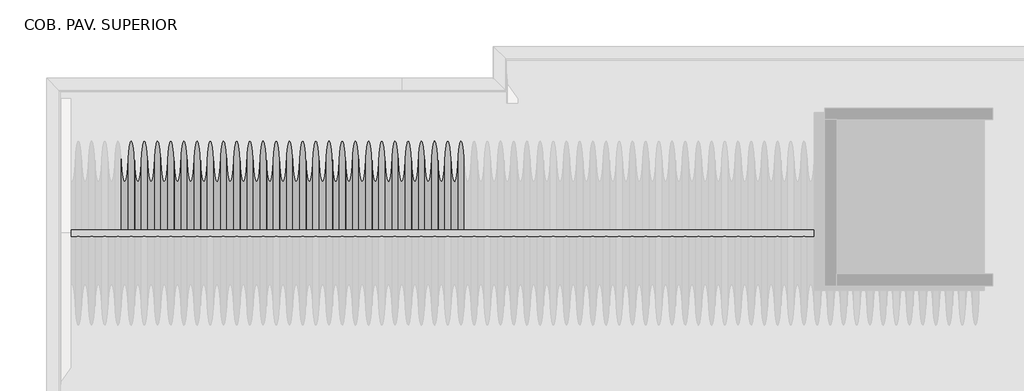
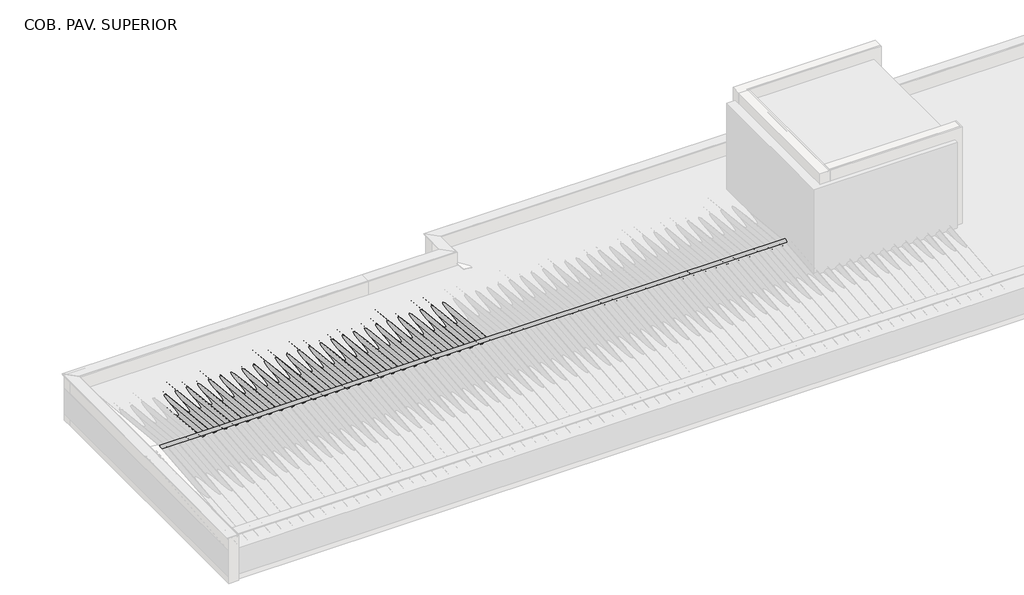
# One storey, part 4 of 8: 36 beams, 8 columns.
"""IFC4 building model written with IfcOpenShell, lengths in millimetres."""

import ifcopenshell
import ifcopenshell.guid

model = None  # the IFC model being written
_history = None  # IfcOwnerHistory: only IFC2X3 demands one
_inside = {}  # id of a spatial element -> (the spatial element, [elements in it])
_under = {}  # id of a project, library or spatial element -> (it, [spatial elements below it])
_declared = {}  # id of a project -> (the project, [libraries it declares])
_typed = {}  # id of a type object -> (the type object, [elements of that type])
_made_of = {}  # id of a material, layer set ... -> (it, [elements and type objects made of it])


def new_model(schema):
    """Start an empty IFC model of exactly this schema.

    Asked for "IFC4X3", IfcOpenShell would pick the latest addendum, in which some entities
    have other attributes; the version numbers below select the first issue.
    IFC2X3 requires an IfcOwnerHistory on every rooted entity: one is made here for all.
    """
    global model, _history
    if schema == "IFC4X3":
        model = ifcopenshell.file(schema_version=(4, 3, 0, 0))
    else:
        model = ifcopenshell.file(schema=schema)
    _inside.clear()
    _under.clear()
    _declared.clear()
    _typed.clear()
    _made_of.clear()
    _history = None
    if model.schema == "IFC2X3":
        org = make("IfcOrganization", Name="unknown")
        user = make(
            "IfcPersonAndOrganization",
            ThePerson=make("IfcPerson", FamilyName="unknown"),
            TheOrganization=org,
        )
        app = make(
            "IfcApplication",
            ApplicationDeveloper=org,
            Version="unknown",
            ApplicationFullName="unknown",
            ApplicationIdentifier="unknown",
        )
        _history = make(
            "IfcOwnerHistory",
            OwningUser=user,
            OwningApplication=app,
            ChangeAction="ADDED",
            CreationDate=0,
        )
    return model


def make(cls, **values):
    """One entity of the class cls with the attributes given. An attribute that is None is left unset."""
    return model.create_entity(
        cls, **{name: value for name, value in values.items() if value is not None}
    )


def rooted(cls, **values):
    """An entity with a GlobalId (a new one), such as an element, a storey or a relation."""
    return make(cls, GlobalId=ifcopenshell.guid.new(), OwnerHistory=_history, **values)


def si_unit(unit_type, name, prefix=None):
    """IfcSIUnit, for example si_unit("LENGTHUNIT", "METRE", prefix="MILLI")."""
    return make("IfcSIUnit", UnitType=unit_type, Prefix=prefix, Name=name)


def assignment(units):
    """IfcUnitAssignment: the units of a project."""
    return None if units is None else make("IfcUnitAssignment", Units=units)


def point(xyz):
    """IfcCartesianPoint."""
    return None if xyz is None else make("IfcCartesianPoint", Coordinates=xyz)


def direction(xyz):
    """IfcDirection."""
    return None if xyz is None else make("IfcDirection", DirectionRatios=xyz)


def frame(location, z_axis=None, x_axis=None):
    """IfcAxis2Placement3D, a coordinate frame: its origin and axes. An axis left out is left unset."""
    return make(
        "IfcAxis2Placement3D",
        Location=point(location),
        Axis=direction(z_axis),
        RefDirection=direction(x_axis),
    )


def frame_2d(location, x_axis=None):
    """IfcAxis2Placement2D, a coordinate frame in the plane: its origin and x axis."""
    return make(
        "IfcAxis2Placement2D", Location=point(location), RefDirection=direction(x_axis)
    )


def origin():
    """The frame at (0, 0, 0) with its axes left unset."""
    return frame((0.0, 0.0, 0.0))


def place(relative_to, where):
    """IfcLocalPlacement: puts the frame where relative to a parent placement (None: the world)."""
    return make(
        "IfcLocalPlacement", PlacementRelTo=relative_to, RelativePlacement=where
    )


def context(
    kind, dimensions, precision=None, world=None, true_north=None, identifier=None
):
    """IfcGeometricRepresentationContext, for example the 3D "Model" context."""
    return make(
        "IfcGeometricRepresentationContext",
        ContextIdentifier=identifier,
        ContextType=kind,
        CoordinateSpaceDimension=dimensions,
        Precision=precision,
        WorldCoordinateSystem=world,
        TrueNorth=true_north,
    )


def project(units=None, contexts=None):
    """IfcProject with its units and contexts."""
    return rooted(
        "IfcProject",
        Name="project",
        RepresentationContexts=contexts,
        UnitsInContext=assignment(units),
    )


def spatial(cls, under=None, at=None, **own):
    """A site, building, storey or space (cls), placed at a placement, below another one or the project."""
    s = rooted(cls, ObjectPlacement=at, **own)
    if under is not None:
        _under.setdefault(under.id(), (under, []))[1].append(s)
    return s


def polyline(points):
    """IfcPolyline through the points."""
    return make("IfcPolyline", Points=[point(p) for p in points])


def circle_curve(where, radius):
    """IfcCircle in the frame where."""
    return make("IfcCircle", Position=where, Radius=radius)


def trimmed(basis, trim1, trim2, sense, master):
    """IfcTrimmedCurve: the piece of a basis curve between two trims."""
    return make(
        "IfcTrimmedCurve",
        BasisCurve=basis,
        Trim1=trim1,
        Trim2=trim2,
        SenseAgreement=sense,
        MasterRepresentation=master,
    )


def segment(curve, same_sense, transition):
    """IfcCompositeCurveSegment."""
    return make(
        "IfcCompositeCurveSegment",
        Transition=transition,
        SameSense=same_sense,
        ParentCurve=curve,
    )


def composite_curve(segments, self_intersect=None):
    """IfcCompositeCurve: segments joined end to end."""
    return make("IfcCompositeCurve", Segments=segments, SelfIntersect=self_intersect)


def outline(outer, holes=None, kind="AREA"):
    """IfcArbitraryClosedProfileDef: a profile drawn as a closed curve; with holes, ...WithVoids."""
    if holes is None:
        return make("IfcArbitraryClosedProfileDef", ProfileType=kind, OuterCurve=outer)
    return make(
        "IfcArbitraryProfileDefWithVoids",
        ProfileType=kind,
        OuterCurve=outer,
        InnerCurves=holes,
    )


def extrude(swept, where, along, depth):
    """IfcExtrudedAreaSolid: the profile swept, set in the frame where, extruded along a direction by depth."""
    return make(
        "IfcExtrudedAreaSolid",
        SweptArea=swept,
        Position=where,
        ExtrudedDirection=direction(along),
        Depth=depth,
    )


def shape(context_of_items, identifier, shape_type, items):
    """IfcShapeRepresentation: the items that make up one representation, for example the "Body"."""
    return make(
        "IfcShapeRepresentation",
        ContextOfItems=context_of_items,
        RepresentationIdentifier=identifier,
        RepresentationType=shape_type,
        Items=items,
    )


def source(mapping_origin, context_of_items, identifier, shape_type, items):
    """IfcRepresentationMap: a shape defined once, which mapped items show again and again."""
    return make(
        "IfcRepresentationMap",
        MappingOrigin=mapping_origin,
        MappedRepresentation=shape(context_of_items, identifier, shape_type, items),
    )


def transform(
    local_origin,
    x_axis=None,
    y_axis=None,
    z_axis=None,
    scale=None,
    scale2=None,
    scale3=None,
    uniform=True,
):
    """IfcCartesianTransformationOperator3D, or its non-uniform kind. x_axis, y_axis, z_axis: its Axis1, 2, 3."""
    if uniform:
        return make(
            "IfcCartesianTransformationOperator3D",
            Axis1=direction(x_axis),
            Axis2=direction(y_axis),
            LocalOrigin=point(local_origin),
            Scale=scale,
            Axis3=direction(z_axis),
        )
    return make(
        "IfcCartesianTransformationOperator3DnonUniform",
        Axis1=direction(x_axis),
        Axis2=direction(y_axis),
        LocalOrigin=point(local_origin),
        Scale=scale,
        Axis3=direction(z_axis),
        Scale2=scale2,
        Scale3=scale3,
    )


def mapped(mapping_source, mapping_target):
    """IfcMappedItem: shows the shape of a source again, moved by a transform."""
    return make(
        "IfcMappedItem", MappingSource=mapping_source, MappingTarget=mapping_target
    )


def made_of(thing, what):
    """Note that an element or type object is made of a material, layer set ...; save() writes the relation."""
    if what is not None:
        _made_of.setdefault(what.id(), (what, []))[1].append(thing)
    return thing


def element(
    cls,
    number,
    at=None,
    inside=None,
    cuts=None,
    type_object=None,
    material=None,
    context=None,
    identifier="Body",
    shape_type=None,
    held_by="IfcProductDefinitionShape",
    body=None,
    shapes=None,
    **own,
):
    """One element of the class cls, such as IfcWall. Its Tag is "e" and its number.

    at: its placement. inside: the storey or other place that contains it. cuts: it is an
    opening in that element (IfcRelVoidsElement). A single representation is given by context,
    identifier, shape_type and body (its items); several are given by shapes. held_by: the class
    of the entity that holds the representations. save() writes the other relations.
    """
    e = rooted(cls, Tag="e%d" % number, ObjectPlacement=at, **own)
    if body is not None:
        shapes = [shape(context, identifier, shape_type, body)]
    if shapes is not None:
        e.Representation = make(held_by, Representations=shapes)
    if inside is not None:
        _inside.setdefault(inside.id(), (inside, []))[1].append(e)
    if cuts is not None:
        rooted(
            "IfcRelVoidsElement", RelatingBuildingElement=cuts, RelatedOpeningElement=e
        )
    if type_object is not None:
        _typed.setdefault(type_object.id(), (type_object, []))[1].append(e)
    return made_of(e, material)


def aggregate(whole, parts):
    """IfcRelAggregates: a whole, such as a stair, and the parts it consists of."""
    return rooted("IfcRelAggregates", RelatingObject=whole, RelatedObjects=parts)


def save(model, path):
    """Write the relations noted so far, then the file.

    IfcRelAggregates (storeys below a building ...), IfcRelContainedInSpatialStructure (elements
    in a storey), IfcRelDefinesByType, IfcRelAssociatesMaterial and IfcRelDeclares: one each for
    every whole, place, type object, material and project.
    """
    for whole, parts in _under.values():
        aggregate(whole, parts)
    for where, things in _inside.values():
        rooted(
            "IfcRelContainedInSpatialStructure",
            RelatedElements=things,
            RelatingStructure=where,
        )
    for kind, things in _typed.values():
        rooted("IfcRelDefinesByType", RelatedObjects=things, RelatingType=kind)
    for what, things in _made_of.values():
        rooted("IfcRelAssociatesMaterial", RelatedObjects=things, RelatingMaterial=what)
    for by, libraries in _declared.values():
        rooted("IfcRelDeclares", RelatingContext=by, RelatedDefinitions=libraries)
    model.write(path)


def beam_fe4ddbad(model_context):
    return source(origin(), model_context, "Body", "SweptSolid", [
        extrude(outline(polyline([(998.8971968, 30.0), (998.8971968, -30.0), (-998.8971974, -30.0), (-998.8971974, 30.0), (998.8971968, 30.0)])), frame((0.0, 0.0, -60.0), z_axis=(0.0, 0.0, 1.0), x_axis=(1.0, 0.0, 0.0)), (0.0, 0.0, 1.0), 120.0),
    ])


def cumeeira_telha_ondulada_fibrocimento_80a8fd81(model_context):
    return source(origin(), model_context, "Body", "SweptSolid", [
        extrude(outline(composite_curve([segment(polyline([(58.3970135, 42.4437972), (53.9055884, 40.2467307)]), True, "CONTINUOUS"), segment(trimmed(circle_curve(frame_2d((-1.6029865, 13.0936483)), 61.7939461), [point((53.9055884, 40.2467307))], [point((-57.1115615, 40.2467307))], True, "CARTESIAN"), True, "CONTINUOUS"), segment(polyline([(-57.1115615, 40.2467307), (-61.6029865, 42.4437972)]), True, "CONTINUOUS"), segment(trimmed(circle_curve(frame_2d((-1.6029865, 13.0936483)), 66.7939461), [point((-61.6029865, 42.4437972))], [point((58.3970135, 42.4437972))], False, "CARTESIAN"), True, "CONTINUOUS")], self_intersect=False)), frame((-7085.3584094, 0.0, 0.0), z_axis=(1.0, 0.0, 0.0), x_axis=(0.0, 1.0, 0.0)), (0.0, 0.0, 1.0), 14170.7168187),
    ])


def viga_cumeeira_6x16cm_bb341ce4(model_context):
    return source(origin(), model_context, "Body", "SweptSolid", [
        extrude(outline(polyline([(7083.3, 30.0), (7083.3, -30.0), (-7082.5, -30.0), (-7082.5, 30.0), (7083.3, 30.0)])), frame((0.0, 0.0, -80.0), z_axis=(0.0, 0.0, 1.0), x_axis=(1.0, 0.0, 0.0)), (0.0, 0.0, 1.0), 160.0),
    ])


def column_6c15bf79(model_context):
    return source(origin(), model_context, "Body", "SweptSolid", [
        extrude(outline(polyline([(30.0, 80.0), (30.0, -80.0), (-30.0, -80.0), (-30.0, 80.0), (30.0, 80.0)])), frame((0.0, 0.0, 6710.0), z_axis=(0.0, 0.0, 1.0), x_axis=(1.0, 0.0, 0.0)), (0.0, 0.0, 1.0), 467.5),
    ])


def column_1adb463a(model_context):
    return source(origin(), model_context, "Body", "SweptSolid", [
        extrude(outline(polyline([(30.0, 80.0), (30.0, -80.0), (-30.0, -80.0), (-30.0, 80.0), (30.0, 80.0)])), frame((0.0, 0.0, 6710.0), z_axis=(0.0, 0.0, 1.0), x_axis=(1.0, 0.0, 0.0)), (0.0, 0.0, 1.0), 284.6),
    ])


def column_910cb117(model_context):
    return source(origin(), model_context, "Body", "SweptSolid", [
        extrude(outline(polyline([(30.0, 80.0), (30.0, -80.0), (-30.0, -80.0), (-30.0, 80.0), (30.0, 80.0)])), frame((0.0, 0.0, 6710.0), z_axis=(0.0, 0.0, 1.0), x_axis=(1.0, 0.0, 0.0)), (0.0, 0.0, 1.0), 371.3),
    ])


model = new_model("IFC4")

# Units and contexts
model_context = context("Model", 3, world=origin())
ifc_project = project(units=[si_unit("LENGTHUNIT", "METRE", prefix="MILLI")], contexts=[model_context])

# Site, building, storey
site = spatial("IfcSite", under=ifc_project)
building = spatial("IfcBuilding", under=site)
storey = spatial("IfcBuildingStorey", under=building, Name="COB. PAV. SUPERIOR", Elevation=6650.0)

# Beams
placement = place(None, origin())
beam_shape = beam_fe4ddbad(model_context)
element("IfcBeam", 1, ObjectType="Madeira de lei : Berço 6x12cm", at=placement, inside=storey, context=model_context, shape_type="MappedRepresentation", body=[
    mapped(beam_shape, transform((-11738.1841096, -6365.3711004, 6680.0), x_axis=(1.0, 0.0, 0.0), y_axis=(0.0, 0.0, -1.0), z_axis=(0.0, 1.0, 0.0))),
])
element("IfcBeam", 2, ObjectType="Madeira de lei : Berço 6x12cm", at=placement, inside=storey, context=model_context, shape_type="MappedRepresentation", body=[
    mapped(beam_shape, transform((-11738.1841096, -5498.3211004, 6680.0), x_axis=(1.0, 0.0, 0.0), y_axis=(0.0, 0.0, -1.0), z_axis=(0.0, 1.0, 0.0))),
])
element("IfcBeam", 3, ObjectType="Madeira de lei : Berço 6x12cm", at=placement, inside=storey, context=model_context, shape_type="MappedRepresentation", body=[
    mapped(beam_shape, transform((-9740.3897147, -7777.6209418, 6680.0), x_axis=(1.0, 0.0, 0.0), y_axis=(0.0, 0.0, -1.0), z_axis=(0.0, 1.0, 0.0))),
])
element("IfcBeam", 4, ObjectType="Madeira de lei : Berço 6x12cm", at=placement, inside=storey, context=model_context, shape_type="MappedRepresentation", body=[
    mapped(beam_shape, transform((-7742.5953199, -7777.6209418, 6680.0), x_axis=(1.0, 0.0, 0.0), y_axis=(0.0, 0.0, -1.0), z_axis=(0.0, 1.0, 0.0))),
])
element("IfcBeam", 5, ObjectType="Madeira de lei : Berço 6x12cm", at=placement, inside=storey, context=model_context, shape_type="MappedRepresentation", body=[
    mapped(beam_shape, transform((-5744.8009251, -7777.6209418, 6680.0), x_axis=(1.0, 0.0, 0.0), y_axis=(0.0, 0.0, -1.0), z_axis=(0.0, 1.0, 0.0))),
])
element("IfcBeam", 6, ObjectType="Madeira de lei : Berço 6x12cm", at=placement, inside=storey, context=model_context, shape_type="MappedRepresentation", body=[
    mapped(beam_shape, transform((-9740.3897147, -6365.3711004, 6680.0), x_axis=(1.0, 0.0, 0.0), y_axis=(0.0, 0.0, -1.0), z_axis=(0.0, 1.0, 0.0))),
])
element("IfcBeam", 7, ObjectType="Madeira de lei : Berço 6x12cm", at=placement, inside=storey, context=model_context, shape_type="MappedRepresentation", body=[
    mapped(beam_shape, transform((-7742.5953199, -6365.3711004, 6680.0), x_axis=(1.0, 0.0, 0.0), y_axis=(0.0, 0.0, -1.0), z_axis=(0.0, 1.0, 0.0))),
])
element("IfcBeam", 8, ObjectType="Madeira de lei : Berço 6x12cm", at=placement, inside=storey, context=model_context, shape_type="MappedRepresentation", body=[
    mapped(beam_shape, transform((-9740.3897147, -5498.3211004, 6680.0), x_axis=(1.0, 0.0, 0.0), y_axis=(0.0, 0.0, -1.0), z_axis=(0.0, 1.0, 0.0))),
])
cumeeira_telha_ondulada_fibrocimento_shape = cumeeira_telha_ondulada_fibrocimento_80a8fd81(model_context)
element("IfcBeam", 9, ObjectType="Cumeeira Telha Ondulada : Fibrocimento", at=placement, inside=storey, context=model_context, shape_type="MappedRepresentation", body=[
    mapped(cumeeira_telha_ondulada_fibrocimento_shape, transform((-5656.9228976, -7777.6209418, 7375.6251229), x_axis=(-1.0, 0.0, 0.0), y_axis=(0.0, -1.0, 0.0), z_axis=(0.0, 0.0, 1.0))),
])
element("IfcBeam", 10, ObjectType="Telha Ondulada : Fibrocimento", at=placement, inside=storey, context=model_context, shape_type="SweptSolid", body=[
    extrude(outline(composite_curve([segment(trimmed(circle_curve(frame_2d((-58.7002978, -53.2060539)), 66.7939461), [point((-29.3501489, 6.7939461))], [point((-29.3501489, -113.2060539))], False, "CARTESIAN"), True, "CONTINUOUS"), segment(polyline([(-29.3501489, -113.2060539), (-31.5472154, -108.7146289)]), True, "CONTINUOUS"), segment(trimmed(circle_curve(frame_2d((-58.7002978, -53.2060539)), 61.7939461), [point((-31.5472154, -108.7146289))], [point((-31.5472154, 2.3025211))], True, "CARTESIAN"), True, "CONTINUOUS"), segment(trimmed(circle_curve(frame_2d((0.0, 66.7939461)), 71.7939461), [point((-31.5472154, 2.3025211))], [point((-31.5472154, 131.2853711))], False, "CARTESIAN"), True, "CONTINUOUS"), segment(polyline([(-31.5472154, 131.2853711), (-29.3501489, 126.7939461)]), True, "CONTINUOUS"), segment(trimmed(circle_curve(frame_2d((0.0, 66.7939461)), 66.7939461), [point((-29.3501489, 126.7939461))], [point((-29.3501489, 6.7939461))], True, "CARTESIAN"), True, "CONTINUOUS")], self_intersect=False)), frame((-11474.7843743, -5298.1805671, 7164.3215886), z_axis=(0.0, -0.9950371902099894, 0.0995037190209978), x_axis=(0.0, 0.0995037190209978, 0.9950371902099894)), (0.0, 0.0, 1.0), 2482.5761317),
])
element("IfcBeam", 11, ObjectType="Telha Ondulada : Fibrocimento", at=placement, inside=storey, context=model_context, shape_type="SweptSolid", body=[
    extrude(outline(composite_curve([segment(trimmed(circle_curve(frame_2d((-58.7002978, -53.2060539)), 66.7939461), [point((-29.3501489, 6.7939461))], [point((-29.3501489, -113.2060539))], False, "CARTESIAN"), True, "CONTINUOUS"), segment(polyline([(-29.3501489, -113.2060539), (-31.5472154, -108.7146289)]), True, "CONTINUOUS"), segment(trimmed(circle_curve(frame_2d((-58.7002978, -53.2060539)), 61.7939461), [point((-31.5472154, -108.7146289))], [point((-31.5472154, 2.3025211))], True, "CARTESIAN"), True, "CONTINUOUS"), segment(trimmed(circle_curve(frame_2d((0.0, 66.7939461)), 71.7939461), [point((-31.5472154, 2.3025211))], [point((-31.5472154, 131.2853711))], False, "CARTESIAN"), True, "CONTINUOUS"), segment(polyline([(-31.5472154, 131.2853711), (-29.3501489, 126.7939461)]), True, "CONTINUOUS"), segment(trimmed(circle_curve(frame_2d((0.0, 66.7939461)), 66.7939461), [point((-29.3501489, 126.7939461))], [point((-29.3501489, 6.7939461))], True, "CARTESIAN"), True, "CONTINUOUS")], self_intersect=False)), frame((-11230.2843743, -5298.1805671, 7164.3215886), z_axis=(0.0, -0.9950371902099894, 0.0995037190209978), x_axis=(0.0, 0.0995037190209978, 0.9950371902099894)), (0.0, 0.0, 1.0), 2482.5761317),
])
element("IfcBeam", 12, ObjectType="Telha Ondulada : Fibrocimento", at=placement, inside=storey, context=model_context, shape_type="SweptSolid", body=[
    extrude(outline(composite_curve([segment(trimmed(circle_curve(frame_2d((-58.7002978, -53.2060539)), 66.7939461), [point((-29.3501489, 6.7939461))], [point((-29.3501489, -113.2060539))], False, "CARTESIAN"), True, "CONTINUOUS"), segment(polyline([(-29.3501489, -113.2060539), (-31.5472154, -108.7146289)]), True, "CONTINUOUS"), segment(trimmed(circle_curve(frame_2d((-58.7002978, -53.2060539)), 61.7939461), [point((-31.5472154, -108.7146289))], [point((-31.5472154, 2.3025211))], True, "CARTESIAN"), True, "CONTINUOUS"), segment(trimmed(circle_curve(frame_2d((0.0, 66.7939461)), 71.7939461), [point((-31.5472154, 2.3025211))], [point((-31.5472154, 131.2853711))], False, "CARTESIAN"), True, "CONTINUOUS"), segment(polyline([(-31.5472154, 131.2853711), (-29.3501489, 126.7939461)]), True, "CONTINUOUS"), segment(trimmed(circle_curve(frame_2d((0.0, 66.7939461)), 66.7939461), [point((-29.3501489, 126.7939461))], [point((-29.3501489, 6.7939461))], True, "CARTESIAN"), True, "CONTINUOUS")], self_intersect=False)), frame((-10985.7843743, -5298.1805671, 7164.3215886), z_axis=(0.0, -0.9950371902099894, 0.09950371902099785), x_axis=(0.0, 0.09950371902099785, 0.9950371902099894)), (0.0, 0.0, 1.0), 2482.5761317),
])
element("IfcBeam", 13, ObjectType="Telha Ondulada : Fibrocimento", at=placement, inside=storey, context=model_context, shape_type="SweptSolid", body=[
    extrude(outline(composite_curve([segment(trimmed(circle_curve(frame_2d((-58.7002978, -53.2060539)), 66.7939461), [point((-29.3501489, 6.7939461))], [point((-29.3501489, -113.2060539))], False, "CARTESIAN"), True, "CONTINUOUS"), segment(polyline([(-29.3501489, -113.2060539), (-31.5472154, -108.7146289)]), True, "CONTINUOUS"), segment(trimmed(circle_curve(frame_2d((-58.7002978, -53.2060539)), 61.7939461), [point((-31.5472154, -108.7146289))], [point((-31.5472154, 2.3025211))], True, "CARTESIAN"), True, "CONTINUOUS"), segment(trimmed(circle_curve(frame_2d((0.0, 66.7939461)), 71.7939461), [point((-31.5472154, 2.3025211))], [point((-31.5472154, 131.2853711))], False, "CARTESIAN"), True, "CONTINUOUS"), segment(polyline([(-31.5472154, 131.2853711), (-29.3501489, 126.7939461)]), True, "CONTINUOUS"), segment(trimmed(circle_curve(frame_2d((0.0, 66.7939461)), 66.7939461), [point((-29.3501489, 126.7939461))], [point((-29.3501489, 6.7939461))], True, "CARTESIAN"), True, "CONTINUOUS")], self_intersect=False)), frame((-10741.2843743, -5298.1805671, 7164.3215886), z_axis=(0.0, -0.9950371902099894, 0.09950371902099785), x_axis=(0.0, 0.09950371902099785, 0.9950371902099894)), (0.0, 0.0, 1.0), 2482.5761317),
])
element("IfcBeam", 14, ObjectType="Telha Ondulada : Fibrocimento", at=placement, inside=storey, context=model_context, shape_type="SweptSolid", body=[
    extrude(outline(composite_curve([segment(trimmed(circle_curve(frame_2d((-58.7002978, -53.2060539)), 66.7939461), [point((-29.3501489, 6.7939461))], [point((-29.3501489, -113.2060539))], False, "CARTESIAN"), True, "CONTINUOUS"), segment(polyline([(-29.3501489, -113.2060539), (-31.5472154, -108.7146289)]), True, "CONTINUOUS"), segment(trimmed(circle_curve(frame_2d((-58.7002978, -53.2060539)), 61.7939461), [point((-31.5472154, -108.7146289))], [point((-31.5472154, 2.3025211))], True, "CARTESIAN"), True, "CONTINUOUS"), segment(trimmed(circle_curve(frame_2d((0.0, 66.7939461)), 71.7939461), [point((-31.5472154, 2.3025211))], [point((-31.5472154, 131.2853711))], False, "CARTESIAN"), True, "CONTINUOUS"), segment(polyline([(-31.5472154, 131.2853711), (-29.3501489, 126.7939461)]), True, "CONTINUOUS"), segment(trimmed(circle_curve(frame_2d((0.0, 66.7939461)), 66.7939461), [point((-29.3501489, 126.7939461))], [point((-29.3501489, 6.7939461))], True, "CARTESIAN"), True, "CONTINUOUS")], self_intersect=False)), frame((-10496.7843743, -5298.1805671, 7164.3215886), z_axis=(0.0, -0.9950371902099894, 0.09950371902099785), x_axis=(0.0, 0.09950371902099785, 0.9950371902099894)), (0.0, 0.0, 1.0), 2482.5761317),
])
element("IfcBeam", 15, ObjectType="Telha Ondulada : Fibrocimento", at=placement, inside=storey, context=model_context, shape_type="SweptSolid", body=[
    extrude(outline(composite_curve([segment(trimmed(circle_curve(frame_2d((-58.7002978, -53.2060539)), 66.7939461), [point((-29.3501489, 6.7939461))], [point((-29.3501489, -113.2060539))], False, "CARTESIAN"), True, "CONTINUOUS"), segment(polyline([(-29.3501489, -113.2060539), (-31.5472154, -108.7146289)]), True, "CONTINUOUS"), segment(trimmed(circle_curve(frame_2d((-58.7002978, -53.2060539)), 61.7939461), [point((-31.5472154, -108.7146289))], [point((-31.5472154, 2.3025211))], True, "CARTESIAN"), True, "CONTINUOUS"), segment(trimmed(circle_curve(frame_2d((0.0, 66.7939461)), 71.7939461), [point((-31.5472154, 2.3025211))], [point((-31.5472154, 131.2853711))], False, "CARTESIAN"), True, "CONTINUOUS"), segment(polyline([(-31.5472154, 131.2853711), (-29.3501489, 126.7939461)]), True, "CONTINUOUS"), segment(trimmed(circle_curve(frame_2d((0.0, 66.7939461)), 66.7939461), [point((-29.3501489, 126.7939461))], [point((-29.3501489, 6.7939461))], True, "CARTESIAN"), True, "CONTINUOUS")], self_intersect=False)), frame((-10252.2843743, -5298.1805671, 7164.3215886), z_axis=(0.0, -0.9950371902099894, 0.09950371902099785), x_axis=(0.0, 0.09950371902099785, 0.9950371902099894)), (0.0, 0.0, 1.0), 2482.5761317),
])
element("IfcBeam", 16, ObjectType="Telha Ondulada : Fibrocimento", at=placement, inside=storey, context=model_context, shape_type="SweptSolid", body=[
    extrude(outline(composite_curve([segment(trimmed(circle_curve(frame_2d((-58.7002978, -53.2060539)), 66.7939461), [point((-29.3501489, 6.7939461))], [point((-29.3501489, -113.2060539))], False, "CARTESIAN"), True, "CONTINUOUS"), segment(polyline([(-29.3501489, -113.2060539), (-31.5472154, -108.7146289)]), True, "CONTINUOUS"), segment(trimmed(circle_curve(frame_2d((-58.7002978, -53.2060539)), 61.7939461), [point((-31.5472154, -108.7146289))], [point((-31.5472154, 2.3025211))], True, "CARTESIAN"), True, "CONTINUOUS"), segment(trimmed(circle_curve(frame_2d((0.0, 66.7939461)), 71.7939461), [point((-31.5472154, 2.3025211))], [point((-31.5472154, 131.2853711))], False, "CARTESIAN"), True, "CONTINUOUS"), segment(polyline([(-31.5472154, 131.2853711), (-29.3501489, 126.7939461)]), True, "CONTINUOUS"), segment(trimmed(circle_curve(frame_2d((0.0, 66.7939461)), 66.7939461), [point((-29.3501489, 126.7939461))], [point((-29.3501489, 6.7939461))], True, "CARTESIAN"), True, "CONTINUOUS")], self_intersect=False)), frame((-10007.7843743, -5298.1805671, 7164.3215886), z_axis=(0.0, -0.9950371902099894, 0.09950371902099785), x_axis=(0.0, 0.09950371902099785, 0.9950371902099894)), (0.0, 0.0, 1.0), 2482.5761317),
])
element("IfcBeam", 17, ObjectType="Telha Ondulada : Fibrocimento", at=placement, inside=storey, context=model_context, shape_type="SweptSolid", body=[
    extrude(outline(composite_curve([segment(trimmed(circle_curve(frame_2d((-58.7002978, -53.2060539)), 66.7939461), [point((-29.3501489, 6.7939461))], [point((-29.3501489, -113.2060539))], False, "CARTESIAN"), True, "CONTINUOUS"), segment(polyline([(-29.3501489, -113.2060539), (-31.5472154, -108.7146289)]), True, "CONTINUOUS"), segment(trimmed(circle_curve(frame_2d((-58.7002978, -53.2060539)), 61.7939461), [point((-31.5472154, -108.7146289))], [point((-31.5472154, 2.3025211))], True, "CARTESIAN"), True, "CONTINUOUS"), segment(trimmed(circle_curve(frame_2d((0.0, 66.7939461)), 71.7939461), [point((-31.5472154, 2.3025211))], [point((-31.5472154, 131.2853711))], False, "CARTESIAN"), True, "CONTINUOUS"), segment(polyline([(-31.5472154, 131.2853711), (-29.3501489, 126.7939461)]), True, "CONTINUOUS"), segment(trimmed(circle_curve(frame_2d((0.0, 66.7939461)), 66.7939461), [point((-29.3501489, 126.7939461))], [point((-29.3501489, 6.7939461))], True, "CARTESIAN"), True, "CONTINUOUS")], self_intersect=False)), frame((-9763.2843743, -5298.1805671, 7164.3215886), z_axis=(0.0, -0.9950371902099894, 0.09950371902099785), x_axis=(0.0, 0.09950371902099785, 0.9950371902099894)), (0.0, 0.0, 1.0), 2482.5761317),
])
element("IfcBeam", 18, ObjectType="Telha Ondulada : Fibrocimento", at=placement, inside=storey, context=model_context, shape_type="SweptSolid", body=[
    extrude(outline(composite_curve([segment(trimmed(circle_curve(frame_2d((-58.7002978, -53.2060539)), 66.7939461), [point((-29.3501489, 6.7939461))], [point((-29.3501489, -113.2060539))], False, "CARTESIAN"), True, "CONTINUOUS"), segment(polyline([(-29.3501489, -113.2060539), (-31.5472154, -108.7146289)]), True, "CONTINUOUS"), segment(trimmed(circle_curve(frame_2d((-58.7002978, -53.2060539)), 61.7939461), [point((-31.5472154, -108.7146289))], [point((-31.5472154, 2.3025211))], True, "CARTESIAN"), True, "CONTINUOUS"), segment(trimmed(circle_curve(frame_2d((0.0, 66.7939461)), 71.7939461), [point((-31.5472154, 2.3025211))], [point((-31.5472154, 131.2853711))], False, "CARTESIAN"), True, "CONTINUOUS"), segment(polyline([(-31.5472154, 131.2853711), (-29.3501489, 126.7939461)]), True, "CONTINUOUS"), segment(trimmed(circle_curve(frame_2d((0.0, 66.7939461)), 66.7939461), [point((-29.3501489, 126.7939461))], [point((-29.3501489, 6.7939461))], True, "CARTESIAN"), True, "CONTINUOUS")], self_intersect=False)), frame((-9518.7843743, -5298.1805671, 7164.3215886), z_axis=(0.0, -0.9950371902099894, 0.09950371902099785), x_axis=(0.0, 0.09950371902099785, 0.9950371902099894)), (0.0, 0.0, 1.0), 2482.5761317),
])
element("IfcBeam", 19, ObjectType="Telha Ondulada : Fibrocimento", at=placement, inside=storey, context=model_context, shape_type="SweptSolid", body=[
    extrude(outline(composite_curve([segment(trimmed(circle_curve(frame_2d((-58.7002978, -53.2060539)), 66.7939461), [point((-29.3501489, 6.7939461))], [point((-29.3501489, -113.2060539))], False, "CARTESIAN"), True, "CONTINUOUS"), segment(polyline([(-29.3501489, -113.2060539), (-31.5472154, -108.7146289)]), True, "CONTINUOUS"), segment(trimmed(circle_curve(frame_2d((-58.7002978, -53.2060539)), 61.7939461), [point((-31.5472154, -108.7146289))], [point((-31.5472154, 2.3025211))], True, "CARTESIAN"), True, "CONTINUOUS"), segment(trimmed(circle_curve(frame_2d((0.0, 66.7939461)), 71.7939461), [point((-31.5472154, 2.3025211))], [point((-31.5472154, 131.2853711))], False, "CARTESIAN"), True, "CONTINUOUS"), segment(polyline([(-31.5472154, 131.2853711), (-29.3501489, 126.7939461)]), True, "CONTINUOUS"), segment(trimmed(circle_curve(frame_2d((0.0, 66.7939461)), 66.7939461), [point((-29.3501489, 126.7939461))], [point((-29.3501489, 6.7939461))], True, "CARTESIAN"), True, "CONTINUOUS")], self_intersect=False)), frame((-9274.2843743, -5298.1805671, 7164.3215886), z_axis=(0.0, -0.9950371902099894, 0.09950371902099785), x_axis=(0.0, 0.09950371902099785, 0.9950371902099894)), (0.0, 0.0, 1.0), 2482.5761317),
])
element("IfcBeam", 20, ObjectType="Telha Ondulada : Fibrocimento", at=placement, inside=storey, context=model_context, shape_type="SweptSolid", body=[
    extrude(outline(composite_curve([segment(trimmed(circle_curve(frame_2d((-58.7002978, -53.2060539)), 66.7939461), [point((-29.3501489, 6.7939461))], [point((-29.3501489, -113.2060539))], False, "CARTESIAN"), True, "CONTINUOUS"), segment(polyline([(-29.3501489, -113.2060539), (-31.5472154, -108.7146289)]), True, "CONTINUOUS"), segment(trimmed(circle_curve(frame_2d((-58.7002978, -53.2060539)), 61.7939461), [point((-31.5472154, -108.7146289))], [point((-31.5472154, 2.3025211))], True, "CARTESIAN"), True, "CONTINUOUS"), segment(trimmed(circle_curve(frame_2d((0.0, 66.7939461)), 71.7939461), [point((-31.5472154, 2.3025211))], [point((-31.5472154, 131.2853711))], False, "CARTESIAN"), True, "CONTINUOUS"), segment(polyline([(-31.5472154, 131.2853711), (-29.3501489, 126.7939461)]), True, "CONTINUOUS"), segment(trimmed(circle_curve(frame_2d((0.0, 66.7939461)), 66.7939461), [point((-29.3501489, 126.7939461))], [point((-29.3501489, 6.7939461))], True, "CARTESIAN"), True, "CONTINUOUS")], self_intersect=False)), frame((-9029.7843743, -5298.1805671, 7164.3215886), z_axis=(0.0, -0.9950371902099894, 0.09950371902099785), x_axis=(0.0, 0.09950371902099785, 0.9950371902099894)), (0.0, 0.0, 1.0), 2482.5761317),
])
element("IfcBeam", 21, ObjectType="Telha Ondulada : Fibrocimento", at=placement, inside=storey, context=model_context, shape_type="SweptSolid", body=[
    extrude(outline(composite_curve([segment(trimmed(circle_curve(frame_2d((-58.7002978, -53.2060539)), 66.7939461), [point((-29.3501489, 6.7939461))], [point((-29.3501489, -113.2060539))], False, "CARTESIAN"), True, "CONTINUOUS"), segment(polyline([(-29.3501489, -113.2060539), (-31.5472154, -108.7146289)]), True, "CONTINUOUS"), segment(trimmed(circle_curve(frame_2d((-58.7002978, -53.2060539)), 61.7939461), [point((-31.5472154, -108.7146289))], [point((-31.5472154, 2.3025211))], True, "CARTESIAN"), True, "CONTINUOUS"), segment(trimmed(circle_curve(frame_2d((0.0, 66.7939461)), 71.7939461), [point((-31.5472154, 2.3025211))], [point((-31.5472154, 131.2853711))], False, "CARTESIAN"), True, "CONTINUOUS"), segment(polyline([(-31.5472154, 131.2853711), (-29.3501489, 126.7939461)]), True, "CONTINUOUS"), segment(trimmed(circle_curve(frame_2d((0.0, 66.7939461)), 66.7939461), [point((-29.3501489, 126.7939461))], [point((-29.3501489, 6.7939461))], True, "CARTESIAN"), True, "CONTINUOUS")], self_intersect=False)), frame((-8785.2843743, -5298.1805671, 7164.3215886), z_axis=(0.0, -0.9950371902099894, 0.09950371902099785), x_axis=(0.0, 0.09950371902099785, 0.9950371902099894)), (0.0, 0.0, 1.0), 2482.5761317),
])
element("IfcBeam", 22, ObjectType="Telha Ondulada : Fibrocimento", at=placement, inside=storey, context=model_context, shape_type="SweptSolid", body=[
    extrude(outline(composite_curve([segment(trimmed(circle_curve(frame_2d((-58.7002978, -53.2060539)), 66.7939461), [point((-29.3501489, 6.7939461))], [point((-29.3501489, -113.2060539))], False, "CARTESIAN"), True, "CONTINUOUS"), segment(polyline([(-29.3501489, -113.2060539), (-31.5472154, -108.7146289)]), True, "CONTINUOUS"), segment(trimmed(circle_curve(frame_2d((-58.7002978, -53.2060539)), 61.7939461), [point((-31.5472154, -108.7146289))], [point((-31.5472154, 2.3025211))], True, "CARTESIAN"), True, "CONTINUOUS"), segment(trimmed(circle_curve(frame_2d((0.0, 66.7939461)), 71.7939461), [point((-31.5472154, 2.3025211))], [point((-31.5472154, 131.2853711))], False, "CARTESIAN"), True, "CONTINUOUS"), segment(polyline([(-31.5472154, 131.2853711), (-29.3501489, 126.7939461)]), True, "CONTINUOUS"), segment(trimmed(circle_curve(frame_2d((0.0, 66.7939461)), 66.7939461), [point((-29.3501489, 126.7939461))], [point((-29.3501489, 6.7939461))], True, "CARTESIAN"), True, "CONTINUOUS")], self_intersect=False)), frame((-8540.7843743, -5298.1805671, 7164.3215886), z_axis=(0.0, -0.9950371902099894, 0.09950371902099785), x_axis=(0.0, 0.09950371902099785, 0.9950371902099894)), (0.0, 0.0, 1.0), 2482.5761317),
])
element("IfcBeam", 23, ObjectType="Telha Ondulada : Fibrocimento", at=placement, inside=storey, context=model_context, shape_type="SweptSolid", body=[
    extrude(outline(composite_curve([segment(trimmed(circle_curve(frame_2d((-58.7002978, -53.2060539)), 66.7939461), [point((-29.3501489, 6.7939461))], [point((-29.3501489, -113.2060539))], False, "CARTESIAN"), True, "CONTINUOUS"), segment(polyline([(-29.3501489, -113.2060539), (-31.5472154, -108.7146289)]), True, "CONTINUOUS"), segment(trimmed(circle_curve(frame_2d((-58.7002978, -53.2060539)), 61.7939461), [point((-31.5472154, -108.7146289))], [point((-31.5472154, 2.3025211))], True, "CARTESIAN"), True, "CONTINUOUS"), segment(trimmed(circle_curve(frame_2d((0.0, 66.7939461)), 71.7939461), [point((-31.5472154, 2.3025211))], [point((-31.5472154, 131.2853711))], False, "CARTESIAN"), True, "CONTINUOUS"), segment(polyline([(-31.5472154, 131.2853711), (-29.3501489, 126.7939461)]), True, "CONTINUOUS"), segment(trimmed(circle_curve(frame_2d((0.0, 66.7939461)), 66.7939461), [point((-29.3501489, 126.7939461))], [point((-29.3501489, 6.7939461))], True, "CARTESIAN"), True, "CONTINUOUS")], self_intersect=False)), frame((-8296.2843743, -5298.1805671, 7164.3215886), z_axis=(0.0, -0.9950371902099894, 0.09950371902099785), x_axis=(0.0, 0.09950371902099785, 0.9950371902099894)), (0.0, 0.0, 1.0), 2482.5761317),
])
element("IfcBeam", 24, ObjectType="Telha Ondulada : Fibrocimento", at=placement, inside=storey, context=model_context, shape_type="SweptSolid", body=[
    extrude(outline(composite_curve([segment(trimmed(circle_curve(frame_2d((-58.7002978, -53.2060539)), 66.7939461), [point((-29.3501489, 6.7939461))], [point((-29.3501489, -113.2060539))], False, "CARTESIAN"), True, "CONTINUOUS"), segment(polyline([(-29.3501489, -113.2060539), (-31.5472154, -108.7146289)]), True, "CONTINUOUS"), segment(trimmed(circle_curve(frame_2d((-58.7002978, -53.2060539)), 61.7939461), [point((-31.5472154, -108.7146289))], [point((-31.5472154, 2.3025211))], True, "CARTESIAN"), True, "CONTINUOUS"), segment(trimmed(circle_curve(frame_2d((0.0, 66.7939461)), 71.7939461), [point((-31.5472154, 2.3025211))], [point((-31.5472154, 131.2853711))], False, "CARTESIAN"), True, "CONTINUOUS"), segment(polyline([(-31.5472154, 131.2853711), (-29.3501489, 126.7939461)]), True, "CONTINUOUS"), segment(trimmed(circle_curve(frame_2d((0.0, 66.7939461)), 66.7939461), [point((-29.3501489, 126.7939461))], [point((-29.3501489, 6.7939461))], True, "CARTESIAN"), True, "CONTINUOUS")], self_intersect=False)), frame((-8051.7843743, -5298.1805671, 7164.3215886), z_axis=(0.0, -0.9950371902099894, 0.0995037190209978), x_axis=(0.0, 0.0995037190209978, 0.9950371902099894)), (0.0, 0.0, 1.0), 2482.5761317),
])
element("IfcBeam", 25, ObjectType="Telha Ondulada : Fibrocimento", at=placement, inside=storey, context=model_context, shape_type="SweptSolid", body=[
    extrude(outline(composite_curve([segment(trimmed(circle_curve(frame_2d((-58.7002978, -53.2060539)), 66.7939461), [point((-29.3501489, 6.7939461))], [point((-29.3501489, -113.2060539))], False, "CARTESIAN"), True, "CONTINUOUS"), segment(polyline([(-29.3501489, -113.2060539), (-31.5472154, -108.7146289)]), True, "CONTINUOUS"), segment(trimmed(circle_curve(frame_2d((-58.7002978, -53.2060539)), 61.7939461), [point((-31.5472154, -108.7146289))], [point((-31.5472154, 2.3025211))], True, "CARTESIAN"), True, "CONTINUOUS"), segment(trimmed(circle_curve(frame_2d((0.0, 66.7939461)), 71.7939461), [point((-31.5472154, 2.3025211))], [point((-31.5472154, 131.2853711))], False, "CARTESIAN"), True, "CONTINUOUS"), segment(polyline([(-31.5472154, 131.2853711), (-29.3501489, 126.7939461)]), True, "CONTINUOUS"), segment(trimmed(circle_curve(frame_2d((0.0, 66.7939461)), 66.7939461), [point((-29.3501489, 126.7939461))], [point((-29.3501489, 6.7939461))], True, "CARTESIAN"), True, "CONTINUOUS")], self_intersect=False)), frame((-7807.2843743, -5298.1805671, 7164.3215886), z_axis=(0.0, -0.9950371902099894, 0.09950371902099785), x_axis=(0.0, 0.09950371902099785, 0.9950371902099894)), (0.0, 0.0, 1.0), 2482.5761317),
])
element("IfcBeam", 26, ObjectType="Telha Ondulada : Fibrocimento", at=placement, inside=storey, context=model_context, shape_type="SweptSolid", body=[
    extrude(outline(composite_curve([segment(trimmed(circle_curve(frame_2d((-58.7002978, -53.2060539)), 66.7939461), [point((-29.3501489, 6.7939461))], [point((-29.3501489, -113.2060539))], False, "CARTESIAN"), True, "CONTINUOUS"), segment(polyline([(-29.3501489, -113.2060539), (-31.5472154, -108.7146289)]), True, "CONTINUOUS"), segment(trimmed(circle_curve(frame_2d((-58.7002978, -53.2060539)), 61.7939461), [point((-31.5472154, -108.7146289))], [point((-31.5472154, 2.3025211))], True, "CARTESIAN"), True, "CONTINUOUS"), segment(trimmed(circle_curve(frame_2d((0.0, 66.7939461)), 71.7939461), [point((-31.5472154, 2.3025211))], [point((-31.5472154, 131.2853711))], False, "CARTESIAN"), True, "CONTINUOUS"), segment(polyline([(-31.5472154, 131.2853711), (-29.3501489, 126.7939461)]), True, "CONTINUOUS"), segment(trimmed(circle_curve(frame_2d((0.0, 66.7939461)), 66.7939461), [point((-29.3501489, 126.7939461))], [point((-29.3501489, 6.7939461))], True, "CARTESIAN"), True, "CONTINUOUS")], self_intersect=False)), frame((-7562.7843743, -5298.1805671, 7164.3215886), z_axis=(0.0, -0.9950371902099894, 0.09950371902099785), x_axis=(0.0, 0.09950371902099785, 0.9950371902099894)), (0.0, 0.0, 1.0), 2482.5761317),
])
element("IfcBeam", 27, ObjectType="Telha Ondulada : Fibrocimento", at=placement, inside=storey, context=model_context, shape_type="SweptSolid", body=[
    extrude(outline(composite_curve([segment(trimmed(circle_curve(frame_2d((-58.7002979, -53.2060539)), 66.7939461), [point((-29.350149, 6.7939461))], [point((-29.350149, -113.2060539))], False, "CARTESIAN"), True, "CONTINUOUS"), segment(polyline([(-29.350149, -113.2060539), (-31.5472155, -108.7146289)]), True, "CONTINUOUS"), segment(trimmed(circle_curve(frame_2d((-58.7002979, -53.2060539)), 61.7939461), [point((-31.5472155, -108.7146289))], [point((-31.5472155, 2.3025211))], True, "CARTESIAN"), True, "CONTINUOUS"), segment(trimmed(circle_curve(frame_2d((0.0, 66.7939461)), 71.7939461), [point((-31.5472155, 2.3025211))], [point((-31.5472155, 131.2853711))], False, "CARTESIAN"), True, "CONTINUOUS"), segment(polyline([(-31.5472155, 131.2853711), (-29.350149, 126.7939461)]), True, "CONTINUOUS"), segment(trimmed(circle_curve(frame_2d((0.0, 66.7939461)), 66.7939461), [point((-29.350149, 126.7939461))], [point((-29.350149, 6.7939461))], True, "CARTESIAN"), True, "CONTINUOUS")], self_intersect=False)), frame((-7318.2843743, -5447.4361457, 7179.2471465), z_axis=(0.0, -0.9950371902099893, 0.09950371902099792), x_axis=(0.0, 0.09950371902099792, 0.9950371902099893)), (0.0, 0.0, 1.0), 2332.5761317),
])
element("IfcBeam", 28, ObjectType="Telha Ondulada : Fibrocimento", at=placement, inside=storey, context=model_context, shape_type="SweptSolid", body=[
    extrude(outline(composite_curve([segment(trimmed(circle_curve(frame_2d((-58.7002978, -53.2060539)), 66.7939461), [point((-29.3501489, 6.7939461))], [point((-29.3501489, -113.2060539))], False, "CARTESIAN"), True, "CONTINUOUS"), segment(polyline([(-29.3501489, -113.2060539), (-31.5472154, -108.7146289)]), True, "CONTINUOUS"), segment(trimmed(circle_curve(frame_2d((-58.7002978, -53.2060539)), 61.7939461), [point((-31.5472154, -108.7146289))], [point((-31.5472154, 2.3025211))], True, "CARTESIAN"), True, "CONTINUOUS"), segment(trimmed(circle_curve(frame_2d((0.0, 66.7939461)), 71.7939461), [point((-31.5472154, 2.3025211))], [point((-31.5472154, 131.2853711))], False, "CARTESIAN"), True, "CONTINUOUS"), segment(polyline([(-31.5472154, 131.2853711), (-29.3501489, 126.7939461)]), True, "CONTINUOUS"), segment(trimmed(circle_curve(frame_2d((0.0, 66.7939461)), 66.7939461), [point((-29.3501489, 126.7939461))], [point((-29.3501489, 6.7939461))], True, "CARTESIAN"), True, "CONTINUOUS")], self_intersect=False)), frame((-7073.7843743, -5298.1805671, 7164.3215886), z_axis=(0.0, -0.9950371902099894, 0.09950371902099785), x_axis=(0.0, 0.09950371902099785, 0.9950371902099894)), (0.0, 0.0, 1.0), 2482.5761317),
])
element("IfcBeam", 29, ObjectType="Telha Ondulada : Fibrocimento", at=placement, inside=storey, context=model_context, shape_type="SweptSolid", body=[
    extrude(outline(composite_curve([segment(trimmed(circle_curve(frame_2d((-58.7002978, -53.2060539)), 66.7939461), [point((-29.3501489, 6.7939461))], [point((-29.3501489, -113.2060539))], False, "CARTESIAN"), True, "CONTINUOUS"), segment(polyline([(-29.3501489, -113.2060539), (-31.5472154, -108.7146289)]), True, "CONTINUOUS"), segment(trimmed(circle_curve(frame_2d((-58.7002978, -53.2060539)), 61.7939461), [point((-31.5472154, -108.7146289))], [point((-31.5472154, 2.3025211))], True, "CARTESIAN"), True, "CONTINUOUS"), segment(trimmed(circle_curve(frame_2d((0.0, 66.7939461)), 71.7939461), [point((-31.5472154, 2.3025211))], [point((-31.5472154, 131.2853711))], False, "CARTESIAN"), True, "CONTINUOUS"), segment(polyline([(-31.5472154, 131.2853711), (-29.3501489, 126.7939461)]), True, "CONTINUOUS"), segment(trimmed(circle_curve(frame_2d((0.0, 66.7939461)), 66.7939461), [point((-29.3501489, 126.7939461))], [point((-29.3501489, 6.7939461))], True, "CARTESIAN"), True, "CONTINUOUS")], self_intersect=False)), frame((-6829.2843743, -5298.1805671, 7164.3215886), z_axis=(0.0, -0.9950371902099894, 0.09950371902099785), x_axis=(0.0, 0.09950371902099785, 0.9950371902099894)), (0.0, 0.0, 1.0), 2482.5761317),
])
element("IfcBeam", 30, ObjectType="Telha Ondulada : Fibrocimento", at=placement, inside=storey, context=model_context, shape_type="SweptSolid", body=[
    extrude(outline(composite_curve([segment(trimmed(circle_curve(frame_2d((-58.7002978, -53.2060539)), 66.7939461), [point((-29.3501489, 6.7939461))], [point((-29.3501489, -113.2060539))], False, "CARTESIAN"), True, "CONTINUOUS"), segment(polyline([(-29.3501489, -113.2060539), (-31.5472154, -108.7146289)]), True, "CONTINUOUS"), segment(trimmed(circle_curve(frame_2d((-58.7002978, -53.2060539)), 61.7939461), [point((-31.5472154, -108.7146289))], [point((-31.5472154, 2.3025211))], True, "CARTESIAN"), True, "CONTINUOUS"), segment(trimmed(circle_curve(frame_2d((0.0, 66.7939461)), 71.7939461), [point((-31.5472154, 2.3025211))], [point((-31.5472154, 131.2853711))], False, "CARTESIAN"), True, "CONTINUOUS"), segment(polyline([(-31.5472154, 131.2853711), (-29.3501489, 126.7939461)]), True, "CONTINUOUS"), segment(trimmed(circle_curve(frame_2d((0.0, 66.7939461)), 66.7939461), [point((-29.3501489, 126.7939461))], [point((-29.3501489, 6.7939461))], True, "CARTESIAN"), True, "CONTINUOUS")], self_intersect=False)), frame((-6584.7843743, -5298.1805671, 7164.3215886), z_axis=(0.0, -0.9950371902099894, 0.09950371902099785), x_axis=(0.0, 0.09950371902099785, 0.9950371902099894)), (0.0, 0.0, 1.0), 2482.5761317),
])
element("IfcBeam", 31, ObjectType="Telha Ondulada : Fibrocimento", at=placement, inside=storey, context=model_context, shape_type="SweptSolid", body=[
    extrude(outline(composite_curve([segment(trimmed(circle_curve(frame_2d((-58.7002978, -53.2060539)), 66.7939461), [point((-29.3501489, 6.7939461))], [point((-29.3501489, -113.2060539))], False, "CARTESIAN"), True, "CONTINUOUS"), segment(polyline([(-29.3501489, -113.2060539), (-31.5472154, -108.7146289)]), True, "CONTINUOUS"), segment(trimmed(circle_curve(frame_2d((-58.7002978, -53.2060539)), 61.7939461), [point((-31.5472154, -108.7146289))], [point((-31.5472154, 2.3025211))], True, "CARTESIAN"), True, "CONTINUOUS"), segment(trimmed(circle_curve(frame_2d((0.0, 66.7939461)), 71.7939461), [point((-31.5472154, 2.3025211))], [point((-31.5472154, 131.2853711))], False, "CARTESIAN"), True, "CONTINUOUS"), segment(polyline([(-31.5472154, 131.2853711), (-29.3501489, 126.7939461)]), True, "CONTINUOUS"), segment(trimmed(circle_curve(frame_2d((0.0, 66.7939461)), 66.7939461), [point((-29.3501489, 126.7939461))], [point((-29.3501489, 6.7939461))], True, "CARTESIAN"), True, "CONTINUOUS")], self_intersect=False)), frame((-6340.2843743, -5298.1805671, 7164.3215886), z_axis=(0.0, -0.9950371902099894, 0.09950371902099785), x_axis=(0.0, 0.09950371902099785, 0.9950371902099894)), (0.0, 0.0, 1.0), 2482.5761317),
])
element("IfcBeam", 32, ObjectType="Telha Ondulada : Fibrocimento", at=placement, inside=storey, context=model_context, shape_type="SweptSolid", body=[
    extrude(outline(composite_curve([segment(trimmed(circle_curve(frame_2d((-58.7002978, -53.2060539)), 66.7939461), [point((-29.3501489, 6.7939461))], [point((-29.3501489, -113.2060539))], False, "CARTESIAN"), True, "CONTINUOUS"), segment(polyline([(-29.3501489, -113.2060539), (-31.5472154, -108.7146289)]), True, "CONTINUOUS"), segment(trimmed(circle_curve(frame_2d((-58.7002978, -53.2060539)), 61.7939461), [point((-31.5472154, -108.7146289))], [point((-31.5472154, 2.3025211))], True, "CARTESIAN"), True, "CONTINUOUS"), segment(trimmed(circle_curve(frame_2d((0.0, 66.7939461)), 71.7939461), [point((-31.5472154, 2.3025211))], [point((-31.5472154, 131.2853711))], False, "CARTESIAN"), True, "CONTINUOUS"), segment(polyline([(-31.5472154, 131.2853711), (-29.3501489, 126.7939461)]), True, "CONTINUOUS"), segment(trimmed(circle_curve(frame_2d((0.0, 66.7939461)), 66.7939461), [point((-29.3501489, 126.7939461))], [point((-29.3501489, 6.7939461))], True, "CARTESIAN"), True, "CONTINUOUS")], self_intersect=False)), frame((-6095.7843743, -5298.1805671, 7164.3215886), z_axis=(0.0, -0.9950371902099894, 0.09950371902099785), x_axis=(0.0, 0.09950371902099785, 0.9950371902099894)), (0.0, 0.0, 1.0), 2482.5761317),
])
element("IfcBeam", 33, ObjectType="Telha Ondulada : Fibrocimento", at=placement, inside=storey, context=model_context, shape_type="SweptSolid", body=[
    extrude(outline(composite_curve([segment(trimmed(circle_curve(frame_2d((-58.7002978, -53.2060539)), 66.7939461), [point((-29.3501489, 6.7939461))], [point((-29.3501489, -113.2060539))], False, "CARTESIAN"), True, "CONTINUOUS"), segment(polyline([(-29.3501489, -113.2060539), (-31.5472154, -108.7146289)]), True, "CONTINUOUS"), segment(trimmed(circle_curve(frame_2d((-58.7002978, -53.2060539)), 61.7939461), [point((-31.5472154, -108.7146289))], [point((-31.5472154, 2.3025211))], True, "CARTESIAN"), True, "CONTINUOUS"), segment(trimmed(circle_curve(frame_2d((0.0, 66.7939461)), 71.7939461), [point((-31.5472154, 2.3025211))], [point((-31.5472154, 131.2853711))], False, "CARTESIAN"), True, "CONTINUOUS"), segment(polyline([(-31.5472154, 131.2853711), (-29.3501489, 126.7939461)]), True, "CONTINUOUS"), segment(trimmed(circle_curve(frame_2d((0.0, 66.7939461)), 66.7939461), [point((-29.3501489, 126.7939461))], [point((-29.3501489, 6.7939461))], True, "CARTESIAN"), True, "CONTINUOUS")], self_intersect=False)), frame((-5851.2843743, -5298.1805671, 7164.3215886), z_axis=(0.0, -0.9950371902099894, 0.09950371902099785), x_axis=(0.0, 0.09950371902099785, 0.9950371902099894)), (0.0, 0.0, 1.0), 2482.5761317),
])
element("IfcBeam", 34, ObjectType="Telha Ondulada : Fibrocimento", at=placement, inside=storey, context=model_context, shape_type="SweptSolid", body=[
    extrude(outline(composite_curve([segment(trimmed(circle_curve(frame_2d((-58.7002978, -53.2060539)), 66.7939461), [point((-29.3501489, 6.7939461))], [point((-29.3501489, -113.2060539))], False, "CARTESIAN"), True, "CONTINUOUS"), segment(polyline([(-29.3501489, -113.2060539), (-31.5472154, -108.7146289)]), True, "CONTINUOUS"), segment(trimmed(circle_curve(frame_2d((-58.7002978, -53.2060539)), 61.7939461), [point((-31.5472154, -108.7146289))], [point((-31.5472154, 2.3025211))], True, "CARTESIAN"), True, "CONTINUOUS"), segment(trimmed(circle_curve(frame_2d((0.0, 66.7939461)), 71.7939461), [point((-31.5472154, 2.3025211))], [point((-31.5472154, 131.2853711))], False, "CARTESIAN"), True, "CONTINUOUS"), segment(polyline([(-31.5472154, 131.2853711), (-29.3501489, 126.7939461)]), True, "CONTINUOUS"), segment(trimmed(circle_curve(frame_2d((0.0, 66.7939461)), 66.7939461), [point((-29.3501489, 126.7939461))], [point((-29.3501489, 6.7939461))], True, "CARTESIAN"), True, "CONTINUOUS")], self_intersect=False)), frame((-5606.7843743, -5298.1805671, 7164.3215886), z_axis=(0.0, -0.9950371902099894, 0.09950371902099785), x_axis=(0.0, 0.09950371902099785, 0.9950371902099894)), (0.0, 0.0, 1.0), 2482.5761317),
])
element("IfcBeam", 35, ObjectType="Telha Ondulada : Fibrocimento", at=placement, inside=storey, context=model_context, shape_type="SweptSolid", body=[
    extrude(outline(composite_curve([segment(trimmed(circle_curve(frame_2d((-58.7002978, -53.2060539)), 66.7939461), [point((-29.3501489, 6.7939461))], [point((-29.3501489, -113.2060539))], False, "CARTESIAN"), True, "CONTINUOUS"), segment(polyline([(-29.3501489, -113.2060539), (-31.5472154, -108.7146289)]), True, "CONTINUOUS"), segment(trimmed(circle_curve(frame_2d((-58.7002978, -53.2060539)), 61.7939461), [point((-31.5472154, -108.7146289))], [point((-31.5472154, 2.3025211))], True, "CARTESIAN"), True, "CONTINUOUS"), segment(trimmed(circle_curve(frame_2d((0.0, 66.7939461)), 71.7939461), [point((-31.5472154, 2.3025211))], [point((-31.5472154, 131.2853711))], False, "CARTESIAN"), True, "CONTINUOUS"), segment(polyline([(-31.5472154, 131.2853711), (-29.3501489, 126.7939461)]), True, "CONTINUOUS"), segment(trimmed(circle_curve(frame_2d((0.0, 66.7939461)), 66.7939461), [point((-29.3501489, 126.7939461))], [point((-29.3501489, 6.7939461))], True, "CARTESIAN"), True, "CONTINUOUS")], self_intersect=False)), frame((-5362.2843743, -5298.1805671, 7164.3215886), z_axis=(0.0, -0.9950371902099894, 0.09950371902099785), x_axis=(0.0, 0.09950371902099785, 0.9950371902099894)), (0.0, 0.0, 1.0), 2482.5761317),
])
viga_cumeeira_6x16cm_shape = viga_cumeeira_6x16cm_bb341ce4(model_context)
element("IfcBeam", 36, ObjectType="Madeira de lei : Viga Cumeeira 6x16cm", at=placement, inside=storey, context=model_context, shape_type="MappedRepresentation", body=[
    mapped(viga_cumeeira_6x16cm_shape, transform((-5654.581307, -7777.6209418, 7258.0), x_axis=(1.0, 0.0, 0.0), y_axis=(0.0, 1.0, 0.0), z_axis=(0.0, 0.0, 1.0))),
])

# Columns
column_shape = column_6c15bf79(model_context)
element("IfcColumn", 37, ObjectType="Madeira de lei-Coluna : Pontalete 6X16cm", at=placement, inside=storey, context=model_context, shape_type="MappedRepresentation", body=[
    mapped(column_shape, transform((-9738.1841096, -7777.6209418, 0.0), x_axis=(0.0, -1.0, 0.0), y_axis=(1.0, 0.0, 0.0), z_axis=(0.0, 0.0, 1.0))),
])
element("IfcColumn", 38, ObjectType="Madeira de lei-Coluna : Pontalete 6X16cm", at=placement, inside=storey, context=model_context, shape_type="MappedRepresentation", body=[
    mapped(column_shape, transform((-7738.1841096, -7777.6209418, 0.0), x_axis=(0.0, -1.0, 0.0), y_axis=(1.0, 0.0, 0.0), z_axis=(0.0, 0.0, 1.0))),
])
element("IfcColumn", 39, ObjectType="Madeira de lei-Coluna : Pontalete 6X16cm", at=placement, inside=storey, context=model_context, shape_type="MappedRepresentation", body=[
    mapped(column_shape, transform((-5738.1841096, -7777.6209418, 0.0), x_axis=(0.0, -1.0, 0.0), y_axis=(1.0, 0.0, 0.0), z_axis=(0.0, 0.0, 1.0))),
])
column_2_shape = column_1adb463a(model_context)
element("IfcColumn", 40, ObjectType="Madeira de lei-Coluna : Pontalete 6X16cm", at=placement, inside=storey, context=model_context, shape_type="MappedRepresentation", body=[
    mapped(column_2_shape, transform((-11738.1841096, -5498.3211004, 0.0), x_axis=(0.0, -1.0, 0.0), y_axis=(1.0, 0.0, 0.0), z_axis=(0.0, 0.0, 1.0))),
])
element("IfcColumn", 41, ObjectType="Madeira de lei-Coluna : Pontalete 6X16cm", at=placement, inside=storey, context=model_context, shape_type="MappedRepresentation", body=[
    mapped(column_2_shape, transform((-9738.1841096, -5498.3211004, 0.0), x_axis=(0.0, -1.0, 0.0), y_axis=(1.0, 0.0, 0.0), z_axis=(0.0, 0.0, 1.0))),
])
column_3_shape = column_910cb117(model_context)
element("IfcColumn", 42, ObjectType="Madeira de lei-Coluna : Pontalete 6X16cm", at=placement, inside=storey, context=model_context, shape_type="MappedRepresentation", body=[
    mapped(column_3_shape, transform((-11738.1841096, -6365.3711004, 0.0), x_axis=(0.0, -1.0, 0.0), y_axis=(1.0, 0.0, 0.0), z_axis=(0.0, 0.0, 1.0))),
])
element("IfcColumn", 43, ObjectType="Madeira de lei-Coluna : Pontalete 6X16cm", at=placement, inside=storey, context=model_context, shape_type="MappedRepresentation", body=[
    mapped(column_3_shape, transform((-9738.1841096, -6365.3711004, 0.0), x_axis=(0.0, -1.0, 0.0), y_axis=(1.0, 0.0, 0.0), z_axis=(0.0, 0.0, 1.0))),
])
element("IfcColumn", 44, ObjectType="Madeira de lei-Coluna : Pontalete 6X16cm", at=placement, inside=storey, context=model_context, shape_type="MappedRepresentation", body=[
    mapped(column_3_shape, transform((-7738.1841096, -6365.3711004, 0.0), x_axis=(0.0, -1.0, 0.0), y_axis=(1.0, 0.0, 0.0), z_axis=(0.0, 0.0, 1.0))),
])

save(model, "model.ifc")

# Revit data of these elements
# Type "Madeira de lei : Berço 6x12cm"
#   A = 0.02 m²
#   Length [instance default] = 1.524 m
#   b = 0.06 m
#   d = 0.12 m
#   Structural Material [instance default] = none
#   Assembly Code = ""
# Type "Cumeeira Telha Ondulada : Fibrocimento"
#   Cost = 5
#   Length [instance default] = 1.524 m
#   b = 0.07 m
#   h = 0.16 m
#   Structural Material = .TELHA DE FIBROCIMENTO
#   Assembly Code = ""
# Type "Telha Ondulada : Fibrocimento"
#   Description = "TELHA ONDULADA FIBROCIMENTO"
#   Cost = 5
#   Length [instance default] = 1.524 m
#   b = 0.07 m
#   h = 0.16 m
#   Structural Material = .TELHA DE FIBROCIMENTO
#   Assembly Code = ""
# Type "Madeira de lei : Viga Cumeeira 6x16cm"
#   A = 0.02 m²
#   Length [instance default] = 1.524 m
#   b = 0.06 m
#   d = 0.16 m
#   Structural Material [instance default] = none
#   Assembly Code = ""
# Type "Madeira de lei-Coluna : Pontalete 6X16cm"
#   A = 0.01952 m²
#   b = 0.06 m
#   d = 0.16 m
#   Structural Material [instance default] = none
#   Assembly Code = ""
# Elements 1, 2, 3, 4, 5, 6, 7, 8 (IfcBeam, "Madeira de lei : Berço 6x12cm")
#   Comments = ""
#   Uso = "TELHADOS ESTRUTURAS"
#   Compr Cmcl = 6.00 m
#   Structural Material = .MADEIRAMENTO
#   Phase Created = CC_AP
#   Materials on its faces: ".MADEIRAMENTO"
# Element 9 (IfcBeam, "Cumeeira Telha Ondulada : Fibrocimento")
#   Comments = ""
#   Uso = "TELHADOS TELHAS"
#   Phase Created = CC_AP
#   Materials on its faces: ".TELHA DE FIBROCIMENTO"
# Elements 10, 11, 12, 13, 14, 15, 16, 17, 18, 19, 20, 21, 22, 23, 24, 25, 26, 27, 28, 29, 30, 31, 32, 33, 34, 35 (IfcBeam, "Telha Ondulada : Fibrocimento")
#   Uso = "TELHADOS TELHAS"
#   Phase Created = CC_AP
#   Materials on its faces: ".TELHA DE FIBROCIMENTO"
# Element 36 (IfcBeam, "Madeira de lei : Viga Cumeeira 6x16cm")
#   Comments = ""
#   Uso = "TELHADOS MADEIRAMENTO"
#   Compr Cmcl = 5.00 m
#   Structural Material = .MADEIRAMENTO
#   Phase Created = CC_AP
#   Materials on its faces: ".MADEIRAMENTO"
# Elements 37, 38, 39 (IfcColumn, "Madeira de lei-Coluna : Pontalete 6X16cm")
#   Comments = ""
#   Uso = "TELHADOS ESTRUTURAS"
#   Compr Cmcl = 6.00 m
#   Structural Material = .MADEIRAMENTO
#   Phase Created = CC_AP
#   Materials on its faces: ".MADEIRAMENTO"
# Elements 40, 41 (IfcColumn, "Madeira de lei-Coluna : Pontalete 6X16cm")
#   Comments = ""
#   Uso = "TELHADOS ESTRUTURAS"
#   Compr Cmcl = 2.00 m
#   Structural Material = .MADEIRAMENTO
#   Phase Created = CC_AP
#   Materials on its faces: ".MADEIRAMENTO"
# Elements 42, 43, 44 (IfcColumn, "Madeira de lei-Coluna : Pontalete 6X16cm")
#   Comments = ""
#   Uso = "TELHADOS ESTRUTURAS"
#   Compr Cmcl = 4.00 m
#   Structural Material = .MADEIRAMENTO
#   Phase Created = CC_AP
#   Materials on its faces: ".MADEIRAMENTO"
# Materials
#   ".TELHA DE FIBROCIMENTO": class "CC_TELHADO", colour RGB 77 77 76, transparency 0, Description = "TELHA ONDULADA FIBROCIMENTO", Cost = 0
#   ".MADEIRAMENTO": class ".CC_MADEIRAS", colour RGB 212 179 113, transparency 0, Cost = 0
